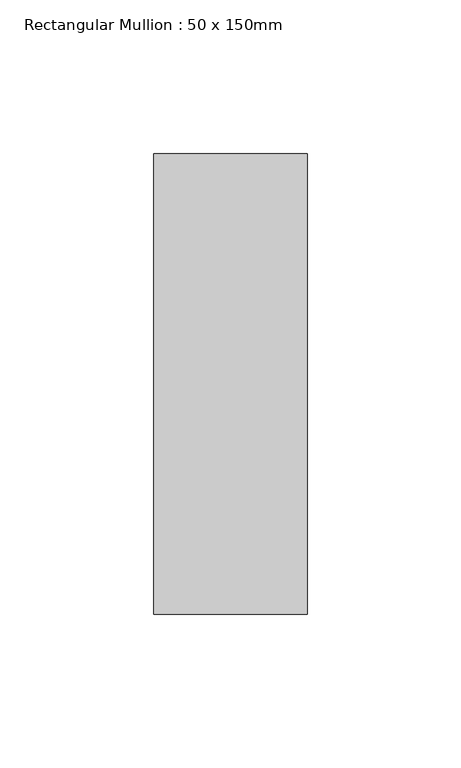
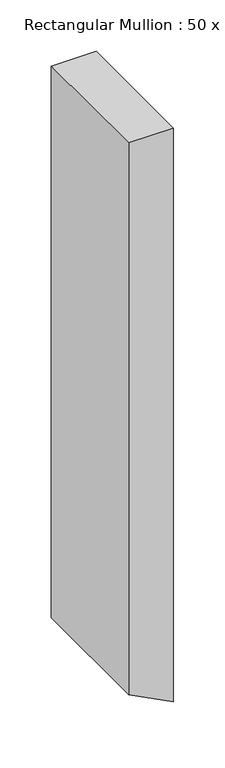
"""IFC4 building model written with IfcOpenShell, lengths in millimetres: member geometry, Rectangular Mullion : 50 x 150mm."""

from ifc_helpers import new_model, si_unit, frame, origin, place, context, project, spatial, polyline, outline, extrude, source, transform, mapped, element, save


def rectangular_mullion_50_x_150mm_fbb4ef83(model_context):
    return source(origin(), model_context, "Body", "SweptSolid", [
        extrude(outline(polyline([(0.0, 0.0), (0.0, -50.0), (-653.8073482, -50.0), (-679.8357007, 0.0), (0.0, 0.0)])), frame((0.0, -75.0, 0.0), z_axis=(0.0, 1.0, 0.0), x_axis=(0.0, 0.0, 1.0)), (0.0, 0.0, 1.0), 150.0),
    ])


if __name__ == "__main__":
    model = new_model("IFC4")
    model_context = context("Model", 3, world=origin())
    ifc_project = project(units=[si_unit("LENGTHUNIT", "METRE", prefix="MILLI")], contexts=[model_context])
    site = spatial("IfcSite", under=ifc_project)
    building = spatial("IfcBuilding", under=site)
    placement = place(None, origin())
    rectangular_mullion_50_x_150mm_shape = rectangular_mullion_50_x_150mm_fbb4ef83(model_context)
    element("IfcMember", 1, ObjectType="Rectangular Mullion : 50 x 150mm", at=placement, inside=building, context=model_context, shape_type="MappedRepresentation", body=[
        mapped(rectangular_mullion_50_x_150mm_shape, transform((0.0, 0.0, 0.0), x_axis=(1.0, 0.0, 0.0), y_axis=(0.0, 1.0, 0.0), z_axis=(0.0, 0.0, 1.0))),
    ])
    save(model, "model.ifc")

# Revit data of these elements
# Type "Rectangular Mullion : 50 x 150mm"
#   built-in parameter 1007304 = 0.492126 (stored number, unit not read)
#   built-in parameter 1007301 = 0.082021 (stored number, unit not read)
#   built-in parameter 1007300 = 0.082021 (stored number, unit not read)
# Element 1 (IfcMember, "Rectangular Mullion : 50 x 150mm")
#   Materials on its faces: "Aluminium"
# Materials
#   "Aluminium": class "Metal", colour RGB 247 247 247, transparency 0, Description = "Aluminium 6061", Cost = 0
